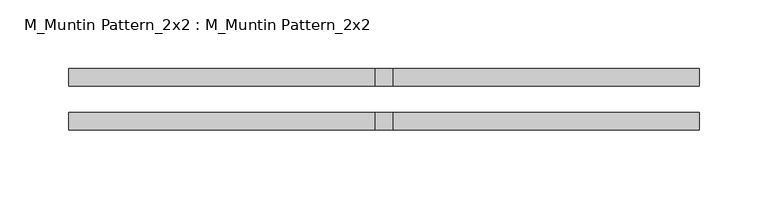
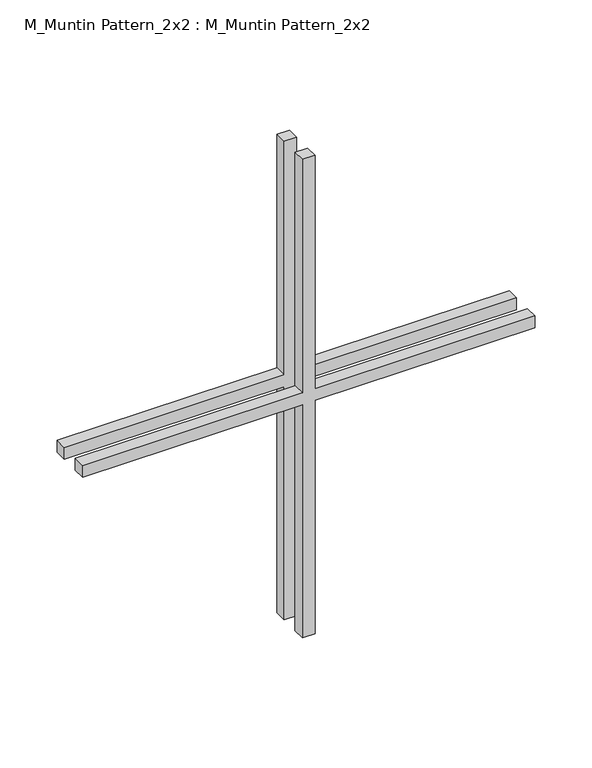
"""IFC4 building model written with IfcOpenShell, lengths in millimetres: proxy geometry, M_Muntin Pattern_2x2 : M_Muntin Pattern_2x2."""

from ifc_helpers import new_model, si_unit, frame, origin, place, context, project, spatial, polyline, outline, extrude, source, transform, mapped, element, save


def m_muntin_pattern_2x2_m_muntin_pattern_2x2_3440c8d2(model_context):
    return source(origin(), model_context, "Body", "SweptSolid", [
        extrude(outline(polyline([(261.9375, -6.35), (261.9375, -228.6), (249.2375, -228.6), (249.2375, -6.35), (0.0, -6.35), (0.0, 6.35), (249.2375, 6.35), (249.2375, 228.6), (261.9375, 228.6), (261.9375, 6.35), (511.175, 6.35), (511.175, -6.35), (261.9375, -6.35)])), frame((0.0, 9.525, 0.0), z_axis=(0.0, 1.0, 0.0), x_axis=(0.0, 0.0, 1.0)), (0.0, 0.0, 1.0), 12.7),
        extrude(outline(polyline([(261.9375, -6.35), (261.9375, -228.6), (249.2375, -228.6), (249.2375, -6.35), (0.0, -6.35), (0.0, 6.35), (249.2375, 6.35), (249.2375, 228.6), (261.9375, 228.6), (261.9375, 6.35), (511.175, 6.35), (511.175, -6.35), (261.9375, -6.35)])), frame((0.0, -22.225, 0.0), z_axis=(0.0, 1.0, 0.0), x_axis=(0.0, 0.0, 1.0)), (0.0, 0.0, 1.0), 12.7),
    ])


if __name__ == "__main__":
    model = new_model("IFC4")
    model_context = context("Model", 3, world=origin())
    ifc_project = project(units=[si_unit("LENGTHUNIT", "METRE", prefix="MILLI")], contexts=[model_context])
    site = spatial("IfcSite", under=ifc_project)
    building = spatial("IfcBuilding", under=site)
    placement = place(None, origin())
    m_muntin_pattern_2x2_m_muntin_pattern_2x2_shape = m_muntin_pattern_2x2_m_muntin_pattern_2x2_3440c8d2(model_context)
    element("IfcBuildingElementProxy", 1, Name="M_Muntin Pattern_2x2 : M_Muntin Pattern_2x2", ObjectType="M_Muntin Pattern_2x2 : M_Muntin Pattern_2x2", at=placement, inside=building, context=model_context, shape_type="MappedRepresentation", body=[
        mapped(m_muntin_pattern_2x2_m_muntin_pattern_2x2_shape, transform((0.0, 0.0, 0.0), x_axis=(1.0, 0.0, 0.0), y_axis=(0.0, 1.0, 0.0), z_axis=(0.0, 0.0, 1.0))),
    ])
    save(model, "model.ifc")

# Revit data of these elements
# Type "M_Muntin Pattern_2x2 : M_Muntin Pattern_2x2"
#   Width [instance default] = 3' - 11.24409"
#   Thickness = 0' - 0 1/2"
#   Height [instance default] = 3' - 11.24409"
#   Distance = 0' - 0 3/4"
#   Interior Material [instance default] = none
#   Exterior Material [instance default] = none
#   Default Elevation = 0
# Element 1 (IfcBuildingElementProxy, "M_Muntin Pattern_2x2 : M_Muntin Pattern_2x2")
#   Width = 1' - 6"
#   Height = 1' - 8 1/8"
#   Interior Material = Wood - Stained
#   Exterior Material = Clad - White
#   Materials on its faces: "Clad - White", "Wood - Stained"
# Materials
#   "Clad - White": class "Wood", colour RGB 242 242 238, transparency 0, Cost = 0
#   "Wood - Stained": class "Wood", colour RGB 224 178 126, transparency 0, Cost = 0
